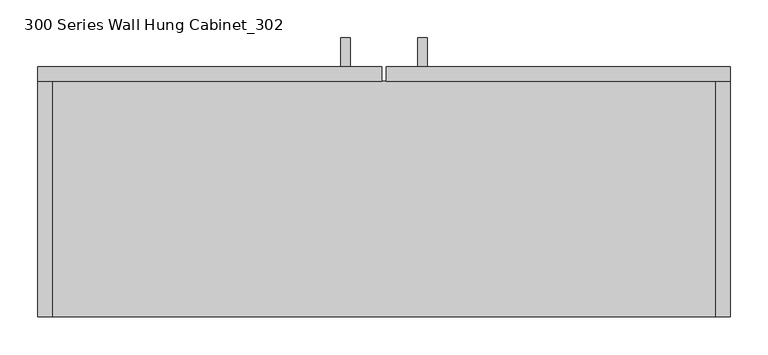
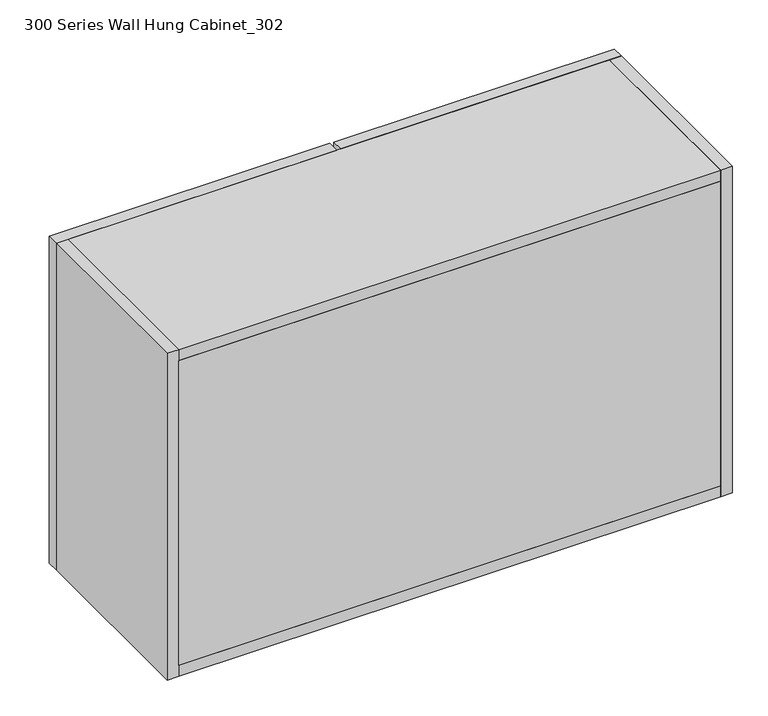
"""IFC4 building model written with IfcOpenShell, lengths in millimetres: furniture geometry, 300 Series Wall Hung Cabinet_302."""

from ifc_helpers import new_model, si_unit, frame, origin, place, context, project, spatial, polyline, outline, extrude, source, transform, mapped, element, save


def furniture_300_series_wall_hung_cabinet_302_8891d94a(model_context):
    return source(origin(), model_context, "Body", "SweptSolid", [
        extrude(outline(polyline([(390.525, 1708.1425373), (390.525, 1720.8121874), (428.6060937, 1720.8121874), (428.6060937, 1625.6), (390.525, 1625.6), (390.525, 1638.2696501), (415.9364436, 1638.2696501), (415.9364436, 1708.1425373), (390.525, 1708.1425373)])), frame((-57.15, 0.0, 0.0), z_axis=(1.0, 0.0, 0.0), x_axis=(0.0, 1.0, 0.0)), (0.0, 0.0, 1.0), 12.4065288),
        extrude(outline(polyline([(390.525, 1708.1425373), (390.525, 1720.8121874), (428.6060937, 1720.8121874), (428.6060937, 1625.6), (390.525, 1625.6), (390.525, 1638.2696501), (415.9364436, 1638.2696501), (415.9364436, 1708.1425373), (390.525, 1708.1425373)])), frame((44.45, 0.0, 0.0), z_axis=(1.0, 0.0, 0.0), x_axis=(0.0, 1.0, 0.0)), (0.0, 0.0, 1.0), 12.4065288),
        extrude(outline(polyline([(438.15, 60.325), (-438.15, 60.325), (-438.15, 79.375), (438.15, 79.375), (438.15, 60.325)])), frame((0.0, 0.0, 1593.85), z_axis=(0.0, 0.0, 1.0), x_axis=(1.0, 0.0, 0.0)), (0.0, 0.0, 1.0), 520.7),
        extrude(outline(polyline([(-3.175, 371.475), (-457.2, 371.475), (-457.2, 390.525), (-3.175, 390.525), (-3.175, 371.475)])), frame((0.0, 0.0, 1574.8), z_axis=(0.0, 0.0, 1.0), x_axis=(1.0, 0.0, 0.0)), (0.0, 0.0, 1.0), 558.8),
        extrude(outline(polyline([(457.2, 371.475), (3.175, 371.475), (3.175, 390.525), (457.2, 390.525), (457.2, 371.475)])), frame((0.0, 0.0, 1574.8), z_axis=(0.0, 0.0, 1.0), x_axis=(1.0, 0.0, 0.0)), (0.0, 0.0, 1.0), 558.8),
        extrude(outline(polyline([(-457.2, 60.325), (-457.2, 371.475), (-438.15, 371.475), (-438.15, 60.325), (-457.2, 60.325)])), frame((0.0, 0.0, 1574.8), z_axis=(0.0, 0.0, 1.0), x_axis=(1.0, 0.0, 0.0)), (0.0, 0.0, 1.0), 558.8),
        extrude(outline(polyline([(438.15, 60.325), (438.15, 371.475), (457.2, 371.475), (457.2, 60.325), (438.15, 60.325)])), frame((0.0, 0.0, 1574.8), z_axis=(0.0, 0.0, 1.0), x_axis=(1.0, 0.0, 0.0)), (0.0, 0.0, 1.0), 558.8),
        extrude(outline(polyline([(438.15, 371.475), (438.15, 60.325), (-438.15, 60.325), (-438.15, 371.475), (438.15, 371.475)])), frame((0.0, 0.0, 2114.55), z_axis=(0.0, 0.0, 1.0), x_axis=(1.0, 0.0, 0.0)), (0.0, 0.0, 1.0), 19.05),
        extrude(outline(polyline([(438.15, 371.475), (438.15, 60.325), (-438.15, 60.325), (-438.15, 371.475), (438.15, 371.475)])), frame((0.0, 0.0, 1574.8), z_axis=(0.0, 0.0, 1.0), x_axis=(1.0, 0.0, 0.0)), (0.0, 0.0, 1.0), 19.05),
    ])


if __name__ == "__main__":
    model = new_model("IFC4")
    model_context = context("Model", 3, world=origin())
    ifc_project = project(units=[si_unit("LENGTHUNIT", "METRE", prefix="MILLI")], contexts=[model_context])
    site = spatial("IfcSite", under=ifc_project)
    building = spatial("IfcBuilding", under=site)
    placement = place(None, origin())
    furniture_300_series_wall_hung_cabinet_302_shape = furniture_300_series_wall_hung_cabinet_302_8891d94a(model_context)
    element("IfcFurniture", 1, ObjectType="300 Series Wall Hung Cabinet_302 : 36\"W x 21\"H", at=placement, inside=building, context=model_context, shape_type="MappedRepresentation", body=[
        mapped(furniture_300_series_wall_hung_cabinet_302_shape, transform((0.0, 0.0, 0.0), x_axis=(1.0, 0.0, 0.0), y_axis=(0.0, 1.0, 0.0), z_axis=(0.0, 0.0, 1.0))),
    ])
    save(model, "model.ifc")

# Revit data of these elements
# Type "300 Series Wall Hung Cabinet_302 : 36\"W x 21\"H"
#   URL = "www.wicnet.org/manual_sections.asp"
#   Model = "302"
#   Manufacturer = "Woodwork Institute"
#   Description = "Wall Hung Cabinet"
#   Content Creator URL = "www.AECcontent.com"
#   Content Creator = "AECcontent"
#   Assembly Code = "E2010200"
#   Width = 3' - 0"
#   Top of Cabinet = 7' - 0"
#   Height = 1' - 10"
#   Depth = 1' - 1"
#   Top Panel Material = none
#   Side Panel Material = none
#   Shelf Panel Material = none
#   Door Panel Material = none
# Element 1 (IfcFurniture, "300 Series Wall Hung Cabinet_302 : 36\"W x 21\"H")
#   Materials on its faces: "CASEWORK"
# Materials
#   "CASEWORK": class "Generic", colour RGB 181 181 181, transparency 0, Cost = 0
